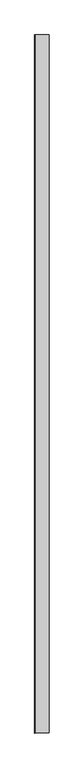
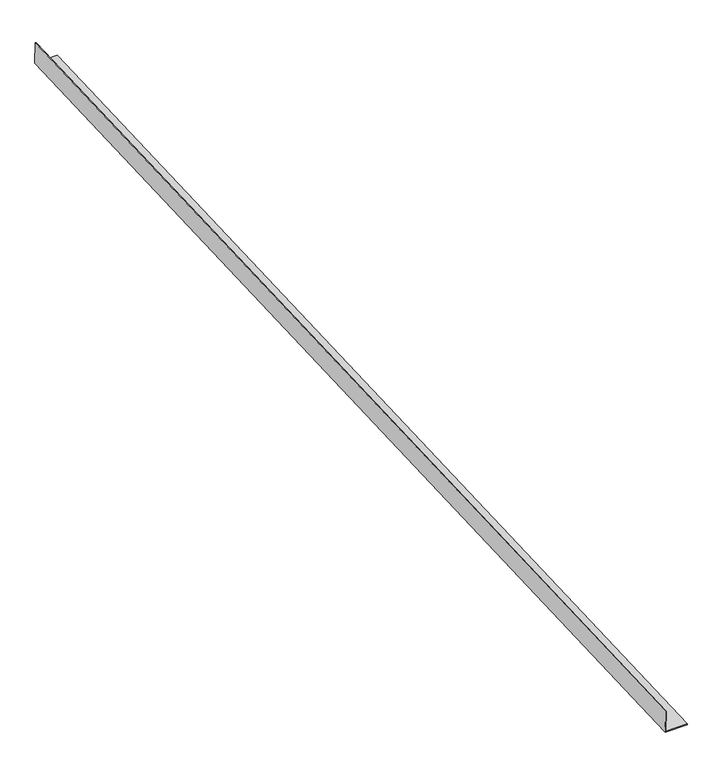
"""IFC4 building model written with IfcOpenShell, lengths in millimetres: proxy geometry, Generic Models 7:Generic Models 1:1:Generic Models 1:1 : Generic Models 7:Generic Models 1:337419:16 : Generic Models 7:Generic Models 1:1:Generic Models 1:1 : Generic Models 7:Generic Models 1:337419:306201."""

from ifc_helpers import new_model, si_unit, frame, origin, place, context, project, spatial, polyline, outline, extrude, source, transform, mapped, element, save


def generic_models_dbb8c6d3(model_context):
    return source(origin(), model_context, "Body", "SweptSolid", [
        extrude(outline(polyline([(101.6, 0.0), (101.6, -101.6), (98.425, -101.6), (98.425, -3.175), (0.0, -3.175), (0.0, 0.0), (101.6, 0.0)])), frame((579304.933599, -578904.4619702, 4198.1978168), z_axis=(0.0, 0.9991330730920964, 0.04163054471831409), x_axis=(0.0, 0.04163054471831409, -0.9991330730920964)), (0.0, 0.0, 1.0), 4955.6806937),
    ])


if __name__ == "__main__":
    model = new_model("IFC4")
    model_context = context("Model", 3, world=origin())
    ifc_project = project(units=[si_unit("LENGTHUNIT", "METRE", prefix="MILLI")], contexts=[model_context])
    site = spatial("IfcSite", under=ifc_project)
    building = spatial("IfcBuilding", under=site)
    placement = place(None, origin())
    generic_models_shape = generic_models_dbb8c6d3(model_context)
    element("IfcBuildingElementProxy", 1, Name="Generic Models 7:Generic Models 1:1:Generic Models 1:1 : Generic Models 7:Generic Models 1:337419:16 : Generic Models 7:Generic Models 1:1:Generic Models 1:1 : Generic Models 7:Generic Models 1:337419:306201", ObjectType="Generic Models 7:Generic Models 1:1:Generic Models 1:1 : Generic Models 7:Generic Models 1:337419:16 : Generic Models 7:Generic Models 1:1:Generic Models 1:1 : Generic Models 7:Generic Models 1:337419:306201", at=placement, inside=building, context=model_context, shape_type="MappedRepresentation", body=[
        mapped(generic_models_shape, transform((0.0, 0.0, 0.0), x_axis=(1.0, 0.0, 0.0), y_axis=(0.0, 1.0, 0.0), z_axis=(0.0, 0.0, 1.0))),
    ])
    save(model, "model.ifc")

# Revit data of these elements
# Type "Generic Models 7:Generic Models 1:1:Generic Models 1:1 : Generic Models 7:Generic Models 1:337419:16 : Generic Models 7:Generic Models 1:1:Generic Models 1:1 : Generic Models 7:Generic Models 1:337419:306201"
#   NameOverride = "Generic Models 7:Generic Models 1:1:Generic Models 1:1 : Generic Models 7:Generic Models 1:337419:306201"
#   ObjectTypeOverride = "Generic Models 1:1 : Generic Models 7:Generic Models 1:337419"
#   Reference = "Generic Models 1"
#   Tag = "306201"
# Element 1 (IfcBuildingElementProxy, "Generic Models 7:Generic Models 1:1:Generic Models 1:1 : Generic Models 7:Generic Models 1:337419:16 : Generic Models 7:Generic Models 1:1:Generic Models 1:1 : Generic Models 7:Generic Models 1:337419:306201")
#   Materials on its faces: "RAKE ANGLE - SEE STRUCT. DWGs"
# Materials
#   "RAKE ANGLE - SEE STRUCT. DWGs": class "Unassigned", colour RGB 210 209 208, transparency 0, Cost = 0
